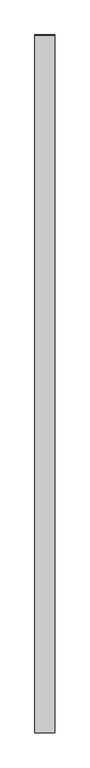
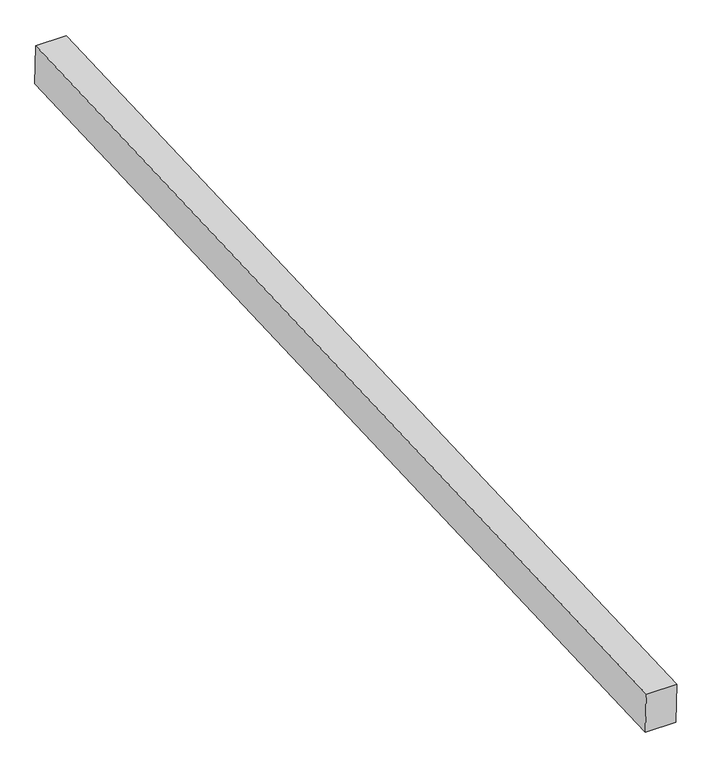
"""IFC4 building model written with IfcOpenShell, lengths in millimetres: proxy geometry, Generic Models 7:Generic Models 1:8:Generic Models 1:8 : Generic Models 7:Generic Models 1:337419:6 : Generic Models 7:Generic Models 1:8:Generic Models 1:8 : Generic Models 7:Generic Models 1:337419:315935."""

from ifc_helpers import new_model, si_unit, frame, origin, place, context, project, spatial, polyline, outline, extrude, source, transform, mapped, element, save


def generic_models_0c9a9326(model_context):
    return source(origin(), model_context, "Body", "SweptSolid", [
        extrude(outline(polyline([(-580524.1699124, 3848.2870208), (-575643.9622189, 4051.6290081), (-575636.3952972, 3861.2790036), (-580516.2392937, 3657.9521704), (-580524.1699124, 3848.2870208)])), frame((593665.061724, 0.0, 0.0), z_axis=(1.0, 0.0, 0.0), x_axis=(0.0, 1.0, 0.0)), (0.0, 0.0, 1.0), 139.7),
    ])


if __name__ == "__main__":
    model = new_model("IFC4")
    model_context = context("Model", 3, world=origin())
    ifc_project = project(units=[si_unit("LENGTHUNIT", "METRE", prefix="MILLI")], contexts=[model_context])
    site = spatial("IfcSite", under=ifc_project)
    building = spatial("IfcBuilding", under=site)
    placement = place(None, origin())
    generic_models_shape = generic_models_0c9a9326(model_context)
    element("IfcBuildingElementProxy", 1, Name="Generic Models 7:Generic Models 1:8:Generic Models 1:8 : Generic Models 7:Generic Models 1:337419:6 : Generic Models 7:Generic Models 1:8:Generic Models 1:8 : Generic Models 7:Generic Models 1:337419:315935", ObjectType="Generic Models 7:Generic Models 1:8:Generic Models 1:8 : Generic Models 7:Generic Models 1:337419:6 : Generic Models 7:Generic Models 1:8:Generic Models 1:8 : Generic Models 7:Generic Models 1:337419:315935", at=placement, inside=building, context=model_context, shape_type="MappedRepresentation", body=[
        mapped(generic_models_shape, transform((0.0, 0.0, 0.0), x_axis=(1.0, 0.0, 0.0), y_axis=(0.0, 1.0, 0.0), z_axis=(0.0, 0.0, 1.0))),
    ])
    save(model, "model.ifc")

# Revit data of these elements
# Type "Generic Models 7:Generic Models 1:8:Generic Models 1:8 : Generic Models 7:Generic Models 1:337419:6 : Generic Models 7:Generic Models 1:8:Generic Models 1:8 : Generic Models 7:Generic Models 1:337419:315935"
#   NameOverride = "Generic Models 7:Generic Models 1:8:Generic Models 1:8 : Generic Models 7:Generic Models 1:337419:315935"
#   ObjectTypeOverride = "Generic Models 1:8 : Generic Models 7:Generic Models 1:337419"
#   Reference = "Generic Models 1"
#   Tag = "315935"
# Element 1 (IfcBuildingElementProxy, "Generic Models 7:Generic Models 1:8:Generic Models 1:8 : Generic Models 7:Generic Models 1:337419:6 : Generic Models 7:Generic Models 1:8:Generic Models 1:8 : Generic Models 7:Generic Models 1:337419:315935")
#   Materials on its faces: "5 1/8\" X 7 1/2\" EXTERIOR GRADE GLULAM BEAMS (4'- 0 1/4\" O.C.)"
# Materials
#   "5 1/8\" X 7 1/2\" EXTERIOR GRADE GLULAM BEAMS (4'- 0 1/4\" O.C.)": class "Wood", colour RGB 183 134 68, transparency 0, Keynote = "M06181300.01", Description = "Pinus Echinata", Cost = 0
